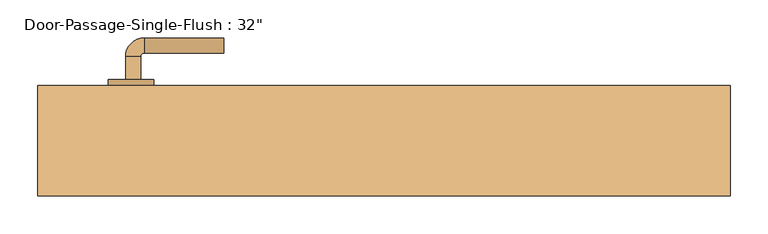
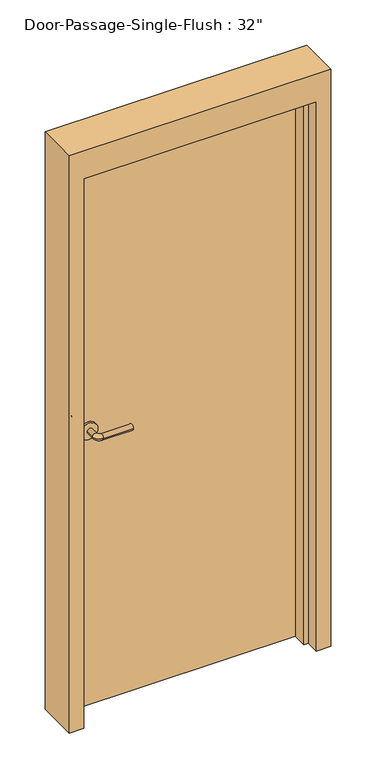
"""IFC4 building model written with IfcOpenShell, lengths in millimetres: door geometry."""

from ifc_helpers import new_model, si_unit, point, frame, frame_2d, origin, origin_with_axes, place, context, project, spatial, polyline, circle_curve, ellipse_curve, trimmed, segment, composite_curve, outline, extrude, faceted_brep, source, transform, mapped, element, save
from ifc_brep_helpers import plane_surface, cylinder_surface, revolved_surface, advanced_brep


def door_8c0afb7b(model_context):
    return source(origin(), model_context, "Body", "SolidModel", [
        advanced_brep(
        [(-341.390625, -3.2375, 1016.0), (-321.390625, -3.2375, 1016.0), (-321.390625, -33.2375, 1016.0), (-341.390625, -33.2375, 1016.0), (-316.390625, -38.2375, 1016.0), (-316.390625, -58.2375, 1016.0), (-211.390625, -58.2375, 1016.0), (-211.390625, -38.2375, 1016.0)],
        [
            (0, 1, circle_curve(frame((-331.390625, -3.2375, 1016.0), z_axis=(0.0, 1.0, 0.0), x_axis=(1.0, 0.0, 0.0)), 10.0)),
            (1, 0, circle_curve(frame((-331.390625, -3.2375, 1016.0), z_axis=(0.0, 1.0, 0.0), x_axis=(1.0, 0.0, 0.0)), 10.0)),
            (1, 2),
            (2, 3, circle_curve(frame((-331.390625, -33.2375, 1016.0), z_axis=(0.0, 1.0, 0.0), x_axis=(1.0, 0.0, 0.0)), 10.0)),
            (3, 0),
            (3, 2, circle_curve(frame((-331.390625, -33.2375, 1016.0), z_axis=(0.0, 1.0, 0.0), x_axis=(1.0, 0.0, 0.0)), 10.0)),
            (4, 5, circle_curve(frame((-316.390625, -48.2375, 1016.0), z_axis=(-1.0, 0.0, 0.0), x_axis=(0.0, 1.0, 0.0)), 10.0)),
            (5, 3, circle_curve(frame((-316.390625, -33.2375, 1016.0), z_axis=(0.0, 0.0, -1.0), x_axis=(-1.0, 0.0, 0.0)), 25.0)),
            (2, 4, circle_curve(frame((-316.390625, -33.2375, 1016.0), z_axis=(0.0, 0.0, 1.0), x_axis=(-1.0, 0.0, 0.0)), 5.0)),
            (5, 4, circle_curve(frame((-316.390625, -48.2375, 1016.0), z_axis=(-1.0, 0.0, 0.0), x_axis=(0.0, 1.0, 0.0)), 10.0)),
            (6, 7, circle_curve(frame((-211.390625, -48.2375, 1016.0), z_axis=(1.0, 0.0, 0.0), x_axis=(0.0, 1.0, 0.0)), 10.0)),
            (7, 6, circle_curve(frame((-211.390625, -48.2375, 1016.0), z_axis=(1.0, 0.0, 0.0), x_axis=(0.0, 1.0, 0.0)), 10.0)),
            (4, 7),
            (6, 5),
        ],
        [
            plane_surface(frame((-331.390625, -3.2375, 1016.0), z_axis=(0.0, 1.0, 0.0), x_axis=(0.0, 0.0, 1.0))),
            cylinder_surface(frame((-331.390625, -3.2375, 1016.0), z_axis=(0.0, 1.0, 0.0), x_axis=(1.0, 0.0, 0.0)), 10.0),
            revolved_surface(trimmed(ellipse_curve(frame((-331.390625, -33.2375, 1016.0), z_axis=(0.0, -1.0, 0.0), x_axis=(1.0, 0.0, 0.0)), 10.0, 10.0), [point((-341.390625, -33.2375, 1016.0))], [point((-321.390625, -33.2375, 1016.0))], True, "CARTESIAN"), (-316.390625, -33.2375, 1016.0), (0.0, 0.0, -1.0)),
            revolved_surface(trimmed(ellipse_curve(frame((-331.390625, -33.2375, 1016.0), z_axis=(0.0, -1.0, 0.0), x_axis=(1.0, 0.0, 0.0)), 10.0, 10.0), [point((-321.390625, -33.2375, 1016.0))], [point((-341.390625, -33.2375, 1016.0))], True, "CARTESIAN"), (-316.390625, -33.2375, 1016.0), (0.0, 0.0, -1.0)),
            plane_surface(frame((-211.390625, -48.2375, 1016.0), z_axis=(1.0, 0.0, 0.0), x_axis=(0.0, 0.0, 1.0))),
            cylinder_surface(frame((-316.390625, -48.2375, 1016.0), z_axis=(-1.0, 0.0, 0.0), x_axis=(0.0, 1.0, 0.0)), 10.0),
        ],
        [
            (0, [[1, 2]]),
            (1, [[3, 4, 5, -2]]),
            (1, [[-5, 6, -3, -1]]),
            (2, [[7, 8, -4, 9]]),
            (3, [[10, -9, -6, -8]]),
            (4, [[11, 12]]),
            (5, [[13, -11, 14, -7]]),
            (5, [[-14, -12, -13, -10]]),
        ],
    ),
        extrude(outline(composite_curve([segment(trimmed(circle_curve(frame_2d((1016.0, -333.890625)), 30.0), [point((1016.0, -363.890625))], [point((1016.0, -303.890625))], False, "CARTESIAN"), True, "CONTINUOUS"), segment(trimmed(circle_curve(frame_2d((1016.0, -333.890625)), 30.0), [point((1016.0, -303.890625))], [point((1016.0, -363.890625))], False, "CARTESIAN"), True, "CONTINUOUS")], self_intersect=False)), frame((0.0, -3.2375, 0.0), z_axis=(0.0, 1.0, 0.0), x_axis=(0.0, 0.0, 1.0)), (0.0, 0.0, 1.0), 8.0),
        advanced_brep(
        [(-341.390625, 57.2125, 1016.0), (-321.390625, 57.2125, 1016.0), (-341.390625, 87.2125, 1016.0), (-321.390625, 87.2125, 1016.0), (-316.390625, 92.2125, 1016.0), (-316.390625, 112.2125, 1016.0), (-211.390625, 112.2125, 1016.0), (-211.390625, 92.2125, 1016.0)],
        [
            (0, 1, circle_curve(frame((-331.390625, 57.2125, 1016.0), z_axis=(0.0, -1.0, 0.0), x_axis=(1.0, 0.0, 0.0)), 10.0)),
            (1, 0, circle_curve(frame((-331.390625, 57.2125, 1016.0), z_axis=(0.0, -1.0, 0.0), x_axis=(1.0, 0.0, 0.0)), 10.0)),
            (0, 2),
            (2, 3, circle_curve(frame((-331.390625, 87.2125, 1016.0), z_axis=(0.0, -1.0, 0.0), x_axis=(1.0, 0.0, 0.0)), 10.0)),
            (3, 1),
            (3, 2, circle_curve(frame((-331.390625, 87.2125, 1016.0), z_axis=(0.0, -1.0, 0.0), x_axis=(1.0, 0.0, 0.0)), 10.0)),
            (4, 3, circle_curve(frame((-316.390625, 87.2125, 1016.0), z_axis=(0.0, 0.0, 1.0), x_axis=(-1.0, 0.0, 0.0)), 5.0)),
            (2, 5, circle_curve(frame((-316.390625, 87.2125, 1016.0), z_axis=(0.0, 0.0, -1.0), x_axis=(-1.0, 0.0, 0.0)), 25.0)),
            (5, 4, circle_curve(frame((-316.390625, 102.2125, 1016.0), z_axis=(-1.0, 0.0, 0.0), x_axis=(0.0, -1.0, 0.0)), 10.0)),
            (4, 5, circle_curve(frame((-316.390625, 102.2125, 1016.0), z_axis=(-1.0, 0.0, 0.0), x_axis=(0.0, -1.0, 0.0)), 10.0)),
            (6, 7, circle_curve(frame((-211.390625, 102.2125, 1016.0), z_axis=(1.0, 0.0, 0.0), x_axis=(0.0, -1.0, 0.0)), 10.0)),
            (7, 6, circle_curve(frame((-211.390625, 102.2125, 1016.0), z_axis=(1.0, 0.0, 0.0), x_axis=(0.0, -1.0, 0.0)), 10.0)),
            (5, 6),
            (7, 4),
        ],
        [
            plane_surface(frame((-331.390625, 57.2125, 1016.0), z_axis=(0.0, -1.0, 0.0), x_axis=(0.0, 0.0, 1.0))),
            cylinder_surface(frame((-331.390625, 57.2125, 1016.0), z_axis=(0.0, -1.0, 0.0), x_axis=(1.0, 0.0, 0.0)), 10.0),
            revolved_surface(trimmed(ellipse_curve(frame((-331.390625, 87.2125, 1016.0), z_axis=(0.0, -1.0, 0.0), x_axis=(1.0, 0.0, 0.0)), 10.0, 10.0), [point((-341.390625, 87.2125, 1016.0))], [point((-321.390625, 87.2125, 1016.0))], True, "CARTESIAN"), (-316.390625, 87.2125, 1016.0), (0.0, 0.0, -1.0)),
            revolved_surface(trimmed(ellipse_curve(frame((-331.390625, 87.2125, 1016.0), z_axis=(0.0, -1.0, 0.0), x_axis=(1.0, 0.0, 0.0)), 10.0, 10.0), [point((-321.390625, 87.2125, 1016.0))], [point((-341.390625, 87.2125, 1016.0))], True, "CARTESIAN"), (-316.390625, 87.2125, 1016.0), (0.0, 0.0, -1.0)),
            plane_surface(frame((-211.390625, 102.2125, 1016.0), z_axis=(1.0, 0.0, 0.0), x_axis=(0.0, 0.0, 1.0))),
            cylinder_surface(frame((-316.390625, 102.2125, 1016.0), z_axis=(-1.0, 0.0, 0.0), x_axis=(0.0, -1.0, 0.0)), 10.0),
        ],
        [
            (0, [[1, 2]]),
            (1, [[-1, 3, 4, 5]]),
            (1, [[-2, -5, 6, -3]]),
            (2, [[7, -4, 8, 9]]),
            (3, [[-8, -6, -7, 10]]),
            (4, [[11, 12]]),
            (5, [[-9, 13, -12, 14]]),
            (5, [[-10, -14, -11, -13]]),
        ],
    ),
        extrude(outline(composite_curve([segment(trimmed(circle_curve(frame_2d((1016.0, -333.890625)), 30.0), [point((1016.0, -363.890625))], [point((1016.0, -303.890625))], False, "CARTESIAN"), True, "CONTINUOUS"), segment(trimmed(circle_curve(frame_2d((1016.0, -333.890625)), 30.0), [point((1016.0, -303.890625))], [point((1016.0, -363.890625))], False, "CARTESIAN"), True, "CONTINUOUS")], self_intersect=False)), frame((0.0, 49.2125, 0.0), z_axis=(0.0, 1.0, 0.0), x_axis=(0.0, 0.0, 1.0)), (0.0, 0.0, 1.0), 8.0),
        faceted_brep([(406.4, 0.0, 0.0), (406.4, 49.2125, 0.0), (457.2, 49.2125, 0.0), (457.2, -96.8375, 0.0), (406.4, -96.8375, 0.0), (406.4, -47.625, 0.0), (390.525, -47.625, 0.0), (390.525, 0.0, 0.0), (406.4, 0.0, 2032.0), (406.4, 49.2125, 2032.0), (-406.4, 49.2125, 2032.0), (-406.4, 49.2125, 0.0), (-457.2, 49.2125, 0.0), (-457.2, 49.2125, 2133.6), (457.2, 49.2125, 2133.6), (457.2, -96.8375, 2133.6), (-457.2, -96.8375, 2133.6), (-457.2, -96.8375, 0.0), (-406.4, -96.8375, 0.0), (-406.4, -96.8375, 2032.0), (406.4, -96.8375, 2032.0), (406.4, -47.625, 2032.0), (-406.4, -47.625, 2032.0), (-406.4, -47.625, 0.0), (-390.525, -47.625, 0.0), (-390.525, -47.625, 2016.125), (390.525, -47.625, 2016.125), (390.525, 0.0, 2016.125), (-390.525, 0.0, 2016.125), (-390.525, 0.0, 0.0), (-406.4, 0.0, 0.0), (-406.4, 0.0, 2032.0)], [[[0, 1, 2, 3, 4, 5, 6, 7]], [[1, 0, 8, 9]], [[2, 1, 9, 10, 11, 12, 13, 14]], [[3, 2, 14, 15]], [[4, 3, 15, 16, 17, 18, 19, 20]], [[5, 4, 20, 21]], [[6, 5, 21, 22, 23, 24, 25, 26]], [[7, 6, 26, 27]], [[0, 7, 27, 28, 29, 30, 31, 8]], [[9, 8, 31, 10]], [[20, 19, 22, 21]], [[26, 25, 28, 27]], [[12, 11, 30, 29, 24, 23, 18, 17]], [[11, 10, 31, 30]], [[13, 12, 17, 16]], [[19, 18, 23, 22]], [[25, 24, 29, 28]], [[15, 14, 13, 16]]]),
        extrude(outline(polyline([(406.4, 4.7625), (-406.4, 4.7625), (-406.4, 49.2125), (406.4, 49.2125), (406.4, 4.7625)])), origin_with_axes(), (0.0, 0.0, 1.0), 2032.0),
    ])


if __name__ == "__main__":
    model = new_model("IFC4")
    model_context = context("Model", 3, world=origin())
    ifc_project = project(units=[si_unit("LENGTHUNIT", "METRE", prefix="MILLI")], contexts=[model_context])
    site = spatial("IfcSite", under=ifc_project)
    building = spatial("IfcBuilding", under=site)
    placement = place(None, origin())
    door_shape = door_8c0afb7b(model_context)
    element("IfcDoor", 1, ObjectType="Door-Passage-Single-Flush : 32\"", at=placement, inside=building, context=model_context, shape_type="MappedRepresentation", body=[
        mapped(door_shape, transform((0.0, 0.0, 0.0), x_axis=(1.0, 0.0, 0.0), y_axis=(0.0, 1.0, 0.0), z_axis=(0.0, 0.0, 1.0))),
    ])
    save(model, "model.ifc")

# Revit data of these elements
# Type "Door-Passage-Single-Flush : 32\""
#   Type Mark = "42"
#   Assembly Code = "B2030200"
#   Analytic Construction = "Wooden"
#   Thickness = 0' - 1 3/4"
#   Thermal Resistance (R) = 0.455703 (m²·K)/W
#   Swing Angle [instance default] = 90.00°
#   Strike Height = 3' - 4"
#   Rough Width [instance default] = 3' - 0"
#   Rough Height [instance default] = 7' - 0"
#   MF Opening Height [instance default] = 0' - 4"
#   MF Opening Width [instance default] = 0' - 4"
#   Inset Calculate [instance default] = 0' - 4"
#   Masonry Inset [instance default] = 0' - 1"
#   Height = 6' - 8"
#   Width = 2' - 8"
#   Heat Transfer Coefficient (U) = 2.19465 W/(m²·K)
#   Masonry Frame Depth = 0' - 5 3/4"
#   Masonry Frame [instance default] = yes
#   Function = 1
#   Dry Wall Frame [instance default] = no
#   Panel Material = Wood - Birch
#   Frame Material = Metal - Paint Finish - Grey
#   Door Handle Material = Aluminum
#   Visual Light Transmittance = 0
#   Solar Heat Gain Coefficient = 0
#   Wall Closure = (empty or 0)
# Element 1 (IfcDoor, "Door-Passage-Single-Flush : 32\"")
#   Materials on its faces: "Aluminum", "Metal - Paint Finish - Grey", "Wood - Birch"
# Materials
#   "Wood - Birch": class "Wood", colour RGB 166 116 52, transparency 0, Cost = 0
#   "Metal - Paint Finish - Grey": class "Paint", colour RGB 104 104 104, transparency 0, Cost = 0
#   "Aluminum": class "Metal", colour RGB 247 247 247, transparency 0, Description = "Aluminum 6061", Cost = 0
